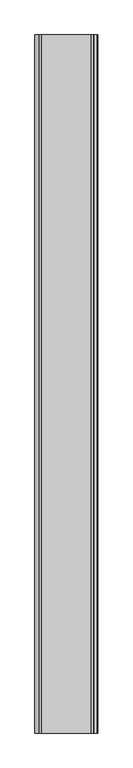
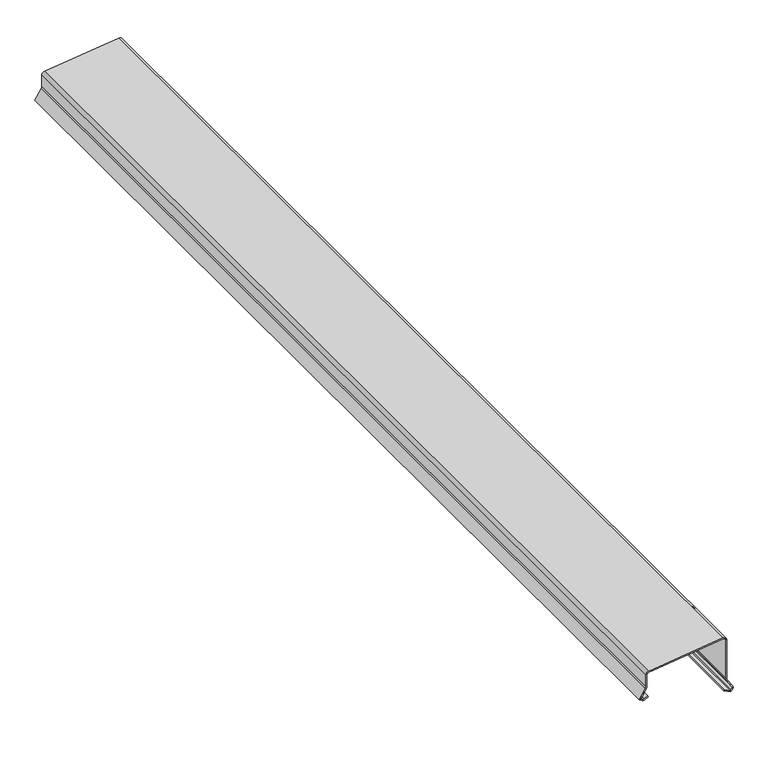
"""IFC4 building model written with IfcOpenShell, lengths in millimetres: proxy geometry, Flashing013 1877 : Flashing013 1877."""

from ifc_helpers import new_model, si_unit, point, frame, frame_2d, origin, place, context, project, spatial, polyline, circle_curve, trimmed, segment, composite_curve, outline, extrude, source, transform, mapped, element, save


def generic_models_fca4859d(model_context):
    return source(origin(), model_context, "Body", "SweptSolid", [
        extrude(outline(composite_curve([segment(polyline([(40127.5360053, -9416.8782953), (40130.8867187, -9409.9548736), (40132.6869689, -9410.8261368), (40129.3362554, -9417.7495585)]), True, "CONTINUOUS"), segment(trimmed(circle_curve(frame_2d((40133.2517994, -9419.6445559)), 4.35), [point((40129.3362554, -9417.7495585))], [point((40129.5632143, -9421.9503831))], True, "CARTESIAN"), True, "CONTINUOUS"), segment(polyline([(40129.5632143, -9421.9503831), (40131.5072723, -9425.0602534), (40148.3948046, -9414.1661265)]), True, "CONTINUOUS"), segment(trimmed(circle_curve(frame_2d((40152.9212544, -9421.1828033)), 8.35), [point((40148.3948046, -9414.1661265))], [point((40152.9212544, -9412.8328033))], False, "CARTESIAN"), True, "CONTINUOUS"), segment(polyline([(40152.9212544, -9412.8328033), (40176.1640916, -9412.8328033)]), True, "CONTINUOUS"), segment(trimmed(circle_curve(frame_2d((40176.1640916, -9408.4828033)), 4.35), [point((40176.1640916, -9412.8328033))], [point((40180.4823161, -9409.0076242))], True, "CARTESIAN"), True, "CONTINUOUS"), segment(polyline([(40180.4823161, -9409.0076242), (40197.712243, -9267.2398508)]), True, "CONTINUOUS"), segment(trimmed(circle_curve(frame_2d((40193.3940184, -9266.7150298)), 4.35), [point((40197.712243, -9267.2398508))], [point((40193.3940184, -9262.3650298))], True, "CARTESIAN"), True, "CONTINUOUS"), segment(polyline([(40193.3940184, -9262.3650298), (40116.1659228, -9262.3650299)]), True, "CONTINUOUS"), segment(trimmed(circle_curve(frame_2d((40116.1659228, -9254.0150299)), 8.35), [point((40116.1659228, -9262.3650299))], [point((40111.6503228, -9261.0386939))], False, "CARTESIAN"), True, "CONTINUOUS"), segment(polyline([(40111.6503228, -9261.0386939), (40095.8098632, -9250.8546675)]), True, "CONTINUOUS"), segment(trimmed(circle_curve(frame_2d((40093.4574249, -9254.5137021)), 4.35), [point((40095.8098632, -9250.8546675))], [point((40089.7935443, -9252.1688185))], True, "CARTESIAN"), True, "CONTINUOUS"), segment(polyline([(40089.7935443, -9252.1688185), (40088.63264, -9253.9827315), (40093.9764738, -9264.6739664), (40092.1875, -9265.5681549), (40086.3359375, -9253.8611236), (40088.1090015, -9251.0907111)]), True, "CONTINUOUS"), segment(trimmed(circle_curve(frame_2d((40093.4574249, -9254.5137021)), 6.35), [point((40088.1090015, -9251.0907111))], [point((40096.8914441, -9249.1723528))], False, "CARTESIAN"), True, "CONTINUOUS"), segment(polyline([(40096.8914441, -9249.1723528), (40112.7319037, -9259.3563791)]), True, "CONTINUOUS"), segment(trimmed(circle_curve(frame_2d((40116.1659228, -9254.0150299)), 6.35), [point((40112.7319037, -9259.3563791))], [point((40116.1659228, -9260.3650299))], True, "CARTESIAN"), True, "CONTINUOUS"), segment(polyline([(40116.1659228, -9260.3650299), (40193.3940184, -9260.3650299)]), True, "CONTINUOUS"), segment(trimmed(circle_curve(frame_2d((40193.3940184, -9266.7150299)), 6.35), [point((40193.3940184, -9260.3650299))], [point((40199.6976336, -9267.4811477))], False, "CARTESIAN"), True, "CONTINUOUS"), segment(polyline([(40199.6976336, -9267.4811477), (40182.4677067, -9409.2489212)]), True, "CONTINUOUS"), segment(trimmed(circle_curve(frame_2d((40176.1640916, -9408.4828033)), 6.35), [point((40182.4677067, -9409.2489212))], [point((40176.1640916, -9414.8328033))], False, "CARTESIAN"), True, "CONTINUOUS"), segment(polyline([(40176.1640916, -9414.8328033), (40152.9212544, -9414.8328033)]), True, "CONTINUOUS"), segment(trimmed(circle_curve(frame_2d((40152.9212544, -9421.1828033)), 6.35), [point((40152.9212544, -9414.8328033))], [point((40149.4789842, -9415.8467677))], True, "CARTESIAN"), True, "CONTINUOUS"), segment(polyline([(40149.4789842, -9415.8467677), (40130.8867187, -9427.8406158), (40127.867313, -9423.0105336)]), True, "CONTINUOUS"), segment(trimmed(circle_curve(frame_2d((40133.2517994, -9419.6445559)), 6.35), [point((40127.867313, -9423.0105336))], [point((40127.5360053, -9416.8782953))], False, "CARTESIAN"), True, "CONTINUOUS")], self_intersect=False)), frame((0.0, 7982.1531721, 0.0), z_axis=(0.0, 1.0, 0.0), x_axis=(0.0, 0.0, 1.0)), (0.0, 0.0, 1.0), 2000.0),
    ])


if __name__ == "__main__":
    model = new_model("IFC4")
    model_context = context("Model", 3, world=origin())
    ifc_project = project(units=[si_unit("LENGTHUNIT", "METRE", prefix="MILLI")], contexts=[model_context])
    site = spatial("IfcSite", under=ifc_project)
    building = spatial("IfcBuilding", under=site)
    placement = place(None, origin())
    generic_models_shape = generic_models_fca4859d(model_context)
    element("IfcBuildingElementProxy", 1, Name="Flashing013 1877 : Flashing013 1877", ObjectType="Flashing013 1877 : Flashing013 1877", at=placement, inside=building, context=model_context, shape_type="MappedRepresentation", body=[
        mapped(generic_models_shape, transform((0.0, 0.0, 0.0), x_axis=(1.0, 0.0, 0.0), y_axis=(0.0, 1.0, 0.0), z_axis=(0.0, 0.0, 1.0))),
    ])
    save(model, "model.ifc")

# Revit data of these elements
# Type "Flashing013 1877 : Flashing013 1877"
#   NameOverride = "Flashing013"
# Element 1 (IfcBuildingElementProxy, "Flashing013 1877 : Flashing013 1877")
#   Materials on its faces: "METAL COPING"
# Materials
#   "METAL COPING": class "Unassigned", colour RGB 128 128 128, transparency 0
